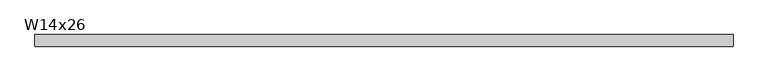
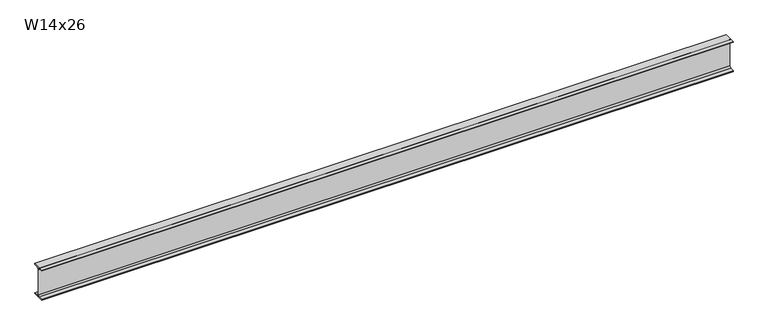
"""IFC4 building model written with IfcOpenShell, lengths in millimetres: beam geometry, RME W-Wide Flange : W14x26."""

from ifc_helpers import new_model, si_unit, point, frame, frame_2d, origin, place, context, project, spatial, polyline, circle_curve, trimmed, segment, composite_curve, outline, extrude, source, transform, mapped, element, save


def w14x26_e8b5ac9c(model_context):
    return source(origin(), model_context, "Body", "SweptSolid", [
        extrude(outline(composite_curve([segment(polyline([(63.881, -165.862), (63.881, -176.53), (-63.881, -176.53), (-63.881, -165.862), (-21.1455, -165.862)]), True, "CONTINUOUS"), segment(trimmed(circle_curve(frame_2d((-21.1455, -147.955)), 17.907), [point((-21.1455, -165.862))], [point((-3.2385, -147.955))], True, "CARTESIAN"), True, "CONTINUOUS"), segment(polyline([(-3.2385, -147.955), (-3.2385, 147.955)]), True, "CONTINUOUS"), segment(trimmed(circle_curve(frame_2d((-21.1455, 147.955)), 17.907), [point((-3.2385, 147.955))], [point((-21.1455, 165.862))], True, "CARTESIAN"), True, "CONTINUOUS"), segment(polyline([(-21.1455, 165.862), (-63.881, 165.862), (-63.881, 176.53), (63.881, 176.53), (63.881, 165.862), (21.1455, 165.862)]), True, "CONTINUOUS"), segment(trimmed(circle_curve(frame_2d((21.1455, 147.955)), 17.907), [point((21.1455, 165.862))], [point((3.2385, 147.955))], True, "CARTESIAN"), True, "CONTINUOUS"), segment(polyline([(3.2385, 147.955), (3.2385, -147.955)]), True, "CONTINUOUS"), segment(trimmed(circle_curve(frame_2d((21.1455, -147.955)), 17.907), [point((3.2385, -147.955))], [point((21.1455, -165.862))], True, "CARTESIAN"), True, "CONTINUOUS"), segment(polyline([(21.1455, -165.862), (63.881, -165.862)]), True, "CONTINUOUS")], self_intersect=False)), frame((-3833.8454775, 0.0, 0.0), z_axis=(1.0, 0.0, 0.0), x_axis=(0.0, 1.0, 0.0)), (0.0, 0.0, 1.0), 7684.6162657),
    ])


if __name__ == "__main__":
    model = new_model("IFC4")
    model_context = context("Model", 3, world=origin())
    ifc_project = project(units=[si_unit("LENGTHUNIT", "METRE", prefix="MILLI")], contexts=[model_context])
    site = spatial("IfcSite", under=ifc_project)
    building = spatial("IfcBuilding", under=site)
    placement = place(None, origin())
    w14x26_shape = w14x26_e8b5ac9c(model_context)
    element("IfcBeam", 1, ObjectType="RME W-Wide Flange : W14x26", at=placement, inside=building, context=model_context, shape_type="MappedRepresentation", body=[
        mapped(w14x26_shape, transform((0.0, 0.0, 0.0), x_axis=(1.0, 0.0, 0.0), y_axis=(0.0, 1.0, 0.0), z_axis=(0.0, 0.0, 1.0))),
    ])
    save(model, "model.ifc")

# Revit data of these elements
# Type "RME W-Wide Flange : W14x26"
#   WELD P [instance default] = ""
#   WELD LE [instance default] = ""
#   WELD D [instance default] = ""
#   TOP SECTION SIZE [instance default] = ""
#   TOP SECTION LENGTH [instance default] = ""
#   REMARKS [instance default] = ""
#   REINF TYPE [instance default] = ""
#   Nominal Size = "W24"
#   End Bearing Capacity [instance default] = ""
#   BOT SECTION SIZE [instance default] = ""
#   BOT SECTION LENGTH [instance default] = ""
#   Assembly Code = "B10"
#   W = 26
#   Start Extension Calculation [instance default] = 10' - 0"
#   Start Extension [instance default] = -0' - 0 1/2"
#   End Extension Calculation [instance default] = 10' - 0"
#   End Extension [instance default] = -0' - 0 1/2"
#   Length [instance default] = 5' - 0"
#   bf = 0' - 5.03"
#   d = 1' - 1.9"
#   k = 0' - 1 1/8"
#   k2 = 0' - 0.705"
#   tf = 0' - 0.42"
#   tw = 0' - 0.255"
#   A = 0.0534028 SF
#   Structural Material [instance default] = Metal - Steel - ASTM A992
# Element 1 (IfcBeam, "RME W-Wide Flange : W14x26")
#   Length = 25' - 11.19031"
#   Materials on its faces: "Metal - Steel - ASTM A992"
# Materials
#   "Metal - Steel - ASTM A992": class "Metal", colour RGB 255 128 0, transparency 0
